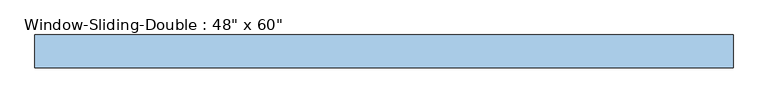
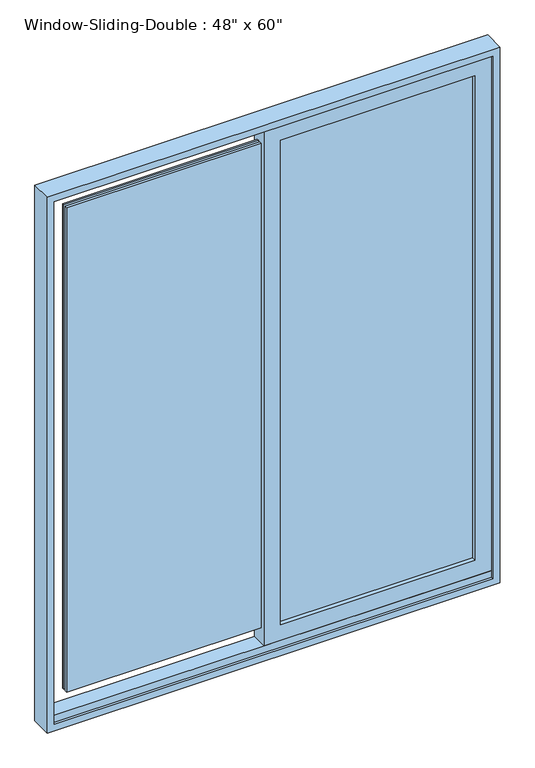
"""IFC4 building model written with IfcOpenShell, lengths in millimetres: window geometry."""

import ifcopenshell
import ifcopenshell.guid

model = None  # the IFC model being written
_history = None  # IfcOwnerHistory: only IFC2X3 demands one
_inside = {}  # id of a spatial element -> (the spatial element, [elements in it])
_under = {}  # id of a project, library or spatial element -> (it, [spatial elements below it])
_declared = {}  # id of a project -> (the project, [libraries it declares])
_typed = {}  # id of a type object -> (the type object, [elements of that type])
_made_of = {}  # id of a material, layer set ... -> (it, [elements and type objects made of it])


def new_model(schema):
    """Start an empty IFC model of exactly this schema.

    Asked for "IFC4X3", IfcOpenShell would pick the latest addendum, in which some entities
    have other attributes; the version numbers below select the first issue.
    IFC2X3 requires an IfcOwnerHistory on every rooted entity: one is made here for all.
    """
    global model, _history
    if schema == "IFC4X3":
        model = ifcopenshell.file(schema_version=(4, 3, 0, 0))
    else:
        model = ifcopenshell.file(schema=schema)
    _inside.clear()
    _under.clear()
    _declared.clear()
    _typed.clear()
    _made_of.clear()
    _history = None
    if model.schema == "IFC2X3":
        org = make("IfcOrganization", Name="unknown")
        user = make(
            "IfcPersonAndOrganization",
            ThePerson=make("IfcPerson", FamilyName="unknown"),
            TheOrganization=org,
        )
        app = make(
            "IfcApplication",
            ApplicationDeveloper=org,
            Version="unknown",
            ApplicationFullName="unknown",
            ApplicationIdentifier="unknown",
        )
        _history = make(
            "IfcOwnerHistory",
            OwningUser=user,
            OwningApplication=app,
            ChangeAction="ADDED",
            CreationDate=0,
        )
    return model


def make(cls, **values):
    """One entity of the class cls with the attributes given. An attribute that is None is left unset."""
    return model.create_entity(
        cls, **{name: value for name, value in values.items() if value is not None}
    )


def rooted(cls, **values):
    """An entity with a GlobalId (a new one), such as an element, a storey or a relation."""
    return make(cls, GlobalId=ifcopenshell.guid.new(), OwnerHistory=_history, **values)


def si_unit(unit_type, name, prefix=None):
    """IfcSIUnit, for example si_unit("LENGTHUNIT", "METRE", prefix="MILLI")."""
    return make("IfcSIUnit", UnitType=unit_type, Prefix=prefix, Name=name)


def assignment(units):
    """IfcUnitAssignment: the units of a project."""
    return None if units is None else make("IfcUnitAssignment", Units=units)


def point(xyz):
    """IfcCartesianPoint."""
    return None if xyz is None else make("IfcCartesianPoint", Coordinates=xyz)


def direction(xyz):
    """IfcDirection."""
    return None if xyz is None else make("IfcDirection", DirectionRatios=xyz)


def frame(location, z_axis=None, x_axis=None):
    """IfcAxis2Placement3D, a coordinate frame: its origin and axes. An axis left out is left unset."""
    return make(
        "IfcAxis2Placement3D",
        Location=point(location),
        Axis=direction(z_axis),
        RefDirection=direction(x_axis),
    )


def origin():
    """The frame at (0, 0, 0) with its axes left unset."""
    return frame((0.0, 0.0, 0.0))


def place(relative_to, where):
    """IfcLocalPlacement: puts the frame where relative to a parent placement (None: the world)."""
    return make(
        "IfcLocalPlacement", PlacementRelTo=relative_to, RelativePlacement=where
    )


def context(
    kind, dimensions, precision=None, world=None, true_north=None, identifier=None
):
    """IfcGeometricRepresentationContext, for example the 3D "Model" context."""
    return make(
        "IfcGeometricRepresentationContext",
        ContextIdentifier=identifier,
        ContextType=kind,
        CoordinateSpaceDimension=dimensions,
        Precision=precision,
        WorldCoordinateSystem=world,
        TrueNorth=true_north,
    )


def project(units=None, contexts=None):
    """IfcProject with its units and contexts."""
    return rooted(
        "IfcProject",
        Name="project",
        RepresentationContexts=contexts,
        UnitsInContext=assignment(units),
    )


def spatial(cls, under=None, at=None, **own):
    """A site, building, storey or space (cls), placed at a placement, below another one or the project."""
    s = rooted(cls, ObjectPlacement=at, **own)
    if under is not None:
        _under.setdefault(under.id(), (under, []))[1].append(s)
    return s


def polyline(points):
    """IfcPolyline through the points."""
    return make("IfcPolyline", Points=[point(p) for p in points])


def outline(outer, holes=None, kind="AREA"):
    """IfcArbitraryClosedProfileDef: a profile drawn as a closed curve; with holes, ...WithVoids."""
    if holes is None:
        return make("IfcArbitraryClosedProfileDef", ProfileType=kind, OuterCurve=outer)
    return make(
        "IfcArbitraryProfileDefWithVoids",
        ProfileType=kind,
        OuterCurve=outer,
        InnerCurves=holes,
    )


def extrude(swept, where, along, depth):
    """IfcExtrudedAreaSolid: the profile swept, set in the frame where, extruded along a direction by depth."""
    return make(
        "IfcExtrudedAreaSolid",
        SweptArea=swept,
        Position=where,
        ExtrudedDirection=direction(along),
        Depth=depth,
    )


def faces_of(points, faces, orient=None, outer=None):
    """IfcFace entities. A face is a list of loops; a loop is a list of indices into points, from 0.

    orient and outer hold one flag for each loop. By default every Orientation is true, the
    first loop of a face is its IfcFaceOuterBound and the others are IfcFaceBound.
    """
    made = []
    for i, loops in enumerate(faces):
        bounds = []
        for j, loop in enumerate(loops):
            is_outer = j == 0 if outer is None else outer[i][j]
            bounds.append(
                make(
                    "IfcFaceOuterBound" if is_outer else "IfcFaceBound",
                    Bound=make("IfcPolyLoop", Polygon=[points[k] for k in loop]),
                    Orientation=True if orient is None else orient[i][j],
                )
            )
        made.append(make("IfcFace", Bounds=bounds))
    return made


def faceted_brep(points, faces, orient=None, outer=None, voids=None):
    """IfcFacetedBrep: a solid bounded by flat faces; with voids (closed shells), ...WithVoids."""
    shared = [point(p) for p in points]
    hull = make("IfcClosedShell", CfsFaces=faces_of(shared, faces, orient, outer))
    if voids is None:
        return make("IfcFacetedBrep", Outer=hull)
    return make(
        "IfcFacetedBrepWithVoids",
        Outer=hull,
        Voids=[
            make(cls, CfsFaces=faces_of(shared, fs, o, b)) for cls, fs, o, b in voids
        ],
    )


def shape(context_of_items, identifier, shape_type, items):
    """IfcShapeRepresentation: the items that make up one representation, for example the "Body"."""
    return make(
        "IfcShapeRepresentation",
        ContextOfItems=context_of_items,
        RepresentationIdentifier=identifier,
        RepresentationType=shape_type,
        Items=items,
    )


def source(mapping_origin, context_of_items, identifier, shape_type, items):
    """IfcRepresentationMap: a shape defined once, which mapped items show again and again."""
    return make(
        "IfcRepresentationMap",
        MappingOrigin=mapping_origin,
        MappedRepresentation=shape(context_of_items, identifier, shape_type, items),
    )


def transform(
    local_origin,
    x_axis=None,
    y_axis=None,
    z_axis=None,
    scale=None,
    scale2=None,
    scale3=None,
    uniform=True,
):
    """IfcCartesianTransformationOperator3D, or its non-uniform kind. x_axis, y_axis, z_axis: its Axis1, 2, 3."""
    if uniform:
        return make(
            "IfcCartesianTransformationOperator3D",
            Axis1=direction(x_axis),
            Axis2=direction(y_axis),
            LocalOrigin=point(local_origin),
            Scale=scale,
            Axis3=direction(z_axis),
        )
    return make(
        "IfcCartesianTransformationOperator3DnonUniform",
        Axis1=direction(x_axis),
        Axis2=direction(y_axis),
        LocalOrigin=point(local_origin),
        Scale=scale,
        Axis3=direction(z_axis),
        Scale2=scale2,
        Scale3=scale3,
    )


def mapped(mapping_source, mapping_target):
    """IfcMappedItem: shows the shape of a source again, moved by a transform."""
    return make(
        "IfcMappedItem", MappingSource=mapping_source, MappingTarget=mapping_target
    )


def made_of(thing, what):
    """Note that an element or type object is made of a material, layer set ...; save() writes the relation."""
    if what is not None:
        _made_of.setdefault(what.id(), (what, []))[1].append(thing)
    return thing


def element(
    cls,
    number,
    at=None,
    inside=None,
    cuts=None,
    type_object=None,
    material=None,
    context=None,
    identifier="Body",
    shape_type=None,
    held_by="IfcProductDefinitionShape",
    body=None,
    shapes=None,
    **own,
):
    """One element of the class cls, such as IfcWall. Its Tag is "e" and its number.

    at: its placement. inside: the storey or other place that contains it. cuts: it is an
    opening in that element (IfcRelVoidsElement). A single representation is given by context,
    identifier, shape_type and body (its items); several are given by shapes. held_by: the class
    of the entity that holds the representations. save() writes the other relations.
    """
    e = rooted(cls, Tag="e%d" % number, ObjectPlacement=at, **own)
    if body is not None:
        shapes = [shape(context, identifier, shape_type, body)]
    if shapes is not None:
        e.Representation = make(held_by, Representations=shapes)
    if inside is not None:
        _inside.setdefault(inside.id(), (inside, []))[1].append(e)
    if cuts is not None:
        rooted(
            "IfcRelVoidsElement", RelatingBuildingElement=cuts, RelatedOpeningElement=e
        )
    if type_object is not None:
        _typed.setdefault(type_object.id(), (type_object, []))[1].append(e)
    return made_of(e, material)


def aggregate(whole, parts):
    """IfcRelAggregates: a whole, such as a stair, and the parts it consists of."""
    return rooted("IfcRelAggregates", RelatingObject=whole, RelatedObjects=parts)


def save(model, path):
    """Write the relations noted so far, then the file.

    IfcRelAggregates (storeys below a building ...), IfcRelContainedInSpatialStructure (elements
    in a storey), IfcRelDefinesByType, IfcRelAssociatesMaterial and IfcRelDeclares: one each for
    every whole, place, type object, material and project.
    """
    for whole, parts in _under.values():
        aggregate(whole, parts)
    for where, things in _inside.values():
        rooted(
            "IfcRelContainedInSpatialStructure",
            RelatedElements=things,
            RelatingStructure=where,
        )
    for kind, things in _typed.values():
        rooted("IfcRelDefinesByType", RelatedObjects=things, RelatingType=kind)
    for what, things in _made_of.values():
        rooted("IfcRelAssociatesMaterial", RelatedObjects=things, RelatingMaterial=what)
    for by, libraries in _declared.values():
        rooted("IfcRelDeclares", RelatingContext=by, RelatedDefinitions=libraries)
    model.write(path)


def window_57c2f901(model_context):
    return source(origin(), model_context, "Body", "SolidModel", [
        faceted_brep([(-609.6, -10.16, 914.4), (-609.6, 46.99, 914.4), (609.6, 46.99, 914.4), (609.6, -10.16, 914.4), (-568.6778905, 46.99, 2397.4778905), (-568.6778905, 40.64, 2397.4778905), (-568.6778905, 40.64, 952.5), (-568.6778905, 40.64, 933.45), (-568.6778905, 46.99, 933.45), (568.6778905, 40.64, 2397.4778905), (568.6778905, 40.64, 952.5), (590.55, 40.64, 952.5), (590.55, 40.64, 2419.35), (-590.55, 40.64, 2419.35), (-590.55, 40.64, 952.5), (-590.55, -10.16, 2419.35), (-590.55, -10.16, 933.45), (-590.55, -3.81, 933.45), (-590.55, -3.81, 952.5), (609.6, -10.16, 2438.4), (-609.6, -10.16, 2438.4), (590.55, -10.16, 2419.35), (590.55, -10.16, 933.45), (-609.6, 46.99, 2438.4), (609.6, 46.99, 2438.4), (568.6778905, 46.99, 933.45), (568.6778905, 46.99, 2397.4778905), (568.6778905, 40.64, 933.45), (590.55, -3.81, 952.5), (590.55, -3.81, 933.45)], [[[0, 1, 2, 3]], [[4, 5, 6, 7, 8]], [[5, 9, 10, 11, 12, 13, 14, 6]], [[13, 15, 16, 17, 18, 14]], [[0, 3, 19, 20], [21, 22, 16, 15]], [[23, 1, 0, 20]], [[2, 1, 23, 24], [4, 8, 25, 26]], [[5, 4, 26, 9]], [[13, 12, 21, 15]], [[20, 19, 24, 23]], [[9, 26, 25, 27, 10]], [[21, 12, 11, 28, 29, 22]], [[19, 3, 2, 24]], [[7, 27, 25, 8]], [[27, 7, 6, 10]], [[10, 6, 14, 18, 28, 11]], [[28, 18, 17, 29]], [[16, 22, 29, 17]]]),
        extrude(outline(polyline([(546.1, 27.94), (546.1, 21.59), (22.225, 21.59), (22.225, 27.94), (546.1, 27.94)])), frame((0.0, 0.0, 996.95), z_axis=(0.0, 0.0, 1.0), x_axis=(1.0, 0.0, 0.0)), (0.0, 0.0, 1.0), 1377.95),
        extrude(outline(polyline([(546.1, 15.24), (546.1, 8.89), (22.225, 8.89), (22.225, 15.24), (546.1, 15.24)])), frame((0.0, 0.0, 996.95), z_axis=(0.0, 0.0, 1.0), x_axis=(1.0, 0.0, 0.0)), (0.0, 0.0, 1.0), 1377.95),
        extrude(outline(polyline([(-22.225, 27.94), (-22.225, 21.59), (-546.1, 21.59), (-546.1, 27.94), (-22.225, 27.94)])), frame((0.0, 0.0, 996.95), z_axis=(0.0, 0.0, 1.0), x_axis=(1.0, 0.0, 0.0)), (0.0, 0.0, 1.0), 1377.95),
        extrude(outline(polyline([(-22.225, 15.24), (-22.225, 8.89), (-546.1, 8.89), (-546.1, 15.24), (-22.225, 15.24)])), frame((0.0, 0.0, 996.95), z_axis=(0.0, 0.0, 1.0), x_axis=(1.0, 0.0, 0.0)), (0.0, 0.0, 1.0), 1377.95),
        extrude(outline(polyline([(952.5, 590.55), (2419.35, 590.55), (2419.35, -22.225), (952.5, -22.225), (952.5, 590.55)]), holes=[polyline([(996.95, 22.225), (2374.9, 22.225), (2374.9, 546.1), (996.95, 546.1), (996.95, 22.225)])]), frame((0.0, -3.81, 0.0), z_axis=(0.0, 1.0, 0.0), x_axis=(0.0, 0.0, 1.0)), (0.0, 0.0, 1.0), 44.45),
    ])


if __name__ == "__main__":
    model = new_model("IFC4")
    model_context = context("Model", 3, world=origin())
    ifc_project = project(units=[si_unit("LENGTHUNIT", "METRE", prefix="MILLI")], contexts=[model_context])
    site = spatial("IfcSite", under=ifc_project)
    building = spatial("IfcBuilding", under=site)
    placement = place(None, origin())
    window_shape = window_57c2f901(model_context)
    element("IfcWindow", 1, ObjectType="Window-Sliding-Double : 48\" x 60\"", at=placement, inside=building, context=model_context, shape_type="MappedRepresentation", body=[
        mapped(window_shape, transform((0.0, 0.0, 0.0), x_axis=(1.0, 0.0, 0.0), y_axis=(0.0, 1.0, 0.0), z_axis=(0.0, 0.0, 1.0))),
    ])
    save(model, "model.ifc")

# Revit data of these elements
# Type "Window-Sliding-Double : 48\" x 60\""
#   Type Mark = "19"
#   Fire Rating = "0.5h"
#   Assembly Code = "B2020100"
#   Analytic Construction = "Double glazing - domestic"
#   Window Inset [instance default] = 0' - 0"
#   Wall Thickness [instance default] = 0' - 6"
#   Visual Light Transmittance = 0.81
#   Thermal Resistance (R) = 1.8146 (h·ft²·°F)/BTU
#   Solar Heat Gain Coefficient = 0.76
#   Muntin Width = 1' - 8 5/8"
#   Muntin Height = 4' - 6 1/4"
#   Interior Wall Closure [instance default] = 0' - 2 3/4"
#   Heat Transfer Coefficient (U) = 0.5511 BTU/(h·ft²·°F)
#   Frame Extension [instance default] = 0' - 0 1/4"
#   Exterior Wall Closure [instance default] = 0' - 1 1/4"
#   Rough Width = 4' - 0 1/2"
#   Rough Height = 5' - 0 1/2"
#   Height = 5' - 0"
#   Extension Jamb [instance default] = 0' - 2 3/4"
#   Default Sill Height = 3' - 0"
#   Width = 4' - 0"
#   Interior Trim Visibility [instance default] = yes
#   Indicator Visibility [instance default] = yes
#   Exterior Trim Visibility [instance default] = yes
#   Muntin Visibility = yes
#   Extension Jamb Visibility [instance default] = yes
#   Muntin Pattern = Muntin Pattern_2x2 : Muntin Pattern_2x2
#   Interior Trim Material = Wood - Stained
#   Interior Trim = Trim-Window-Interior-Flat : Picture Frame
#   Interior Frame Material = Wood - Stained
#   Glass Panel Material = Glass
#   Exterior Trim Material = Clad - White
#   Exterior Trim = Trim-Window-Exterior-Flat : with Sill
#   Exterior Frame Material = Clad - White
#   Wall Closure = (empty or 0)
# Element 1 (IfcWindow, "Window-Sliding-Double : 48\" x 60\"")
#   Wall Thickness = 0' - 2 1/2"
#   Extension Jamb = 0' - 1"
#   Extension Jamb Visibility = no
#   Materials on its faces: "Glass", "Wood - Stained", "Clad - White"
# Materials
#   "Wood - Stained": class "Wood", colour RGB 224 178 126, transparency 0, Cost = 0
#   "Glass": class "Glass", colour RGB 0 128 192, transparency 0.75, Description = "Soda Lime Glass", Cost = 0
#   "Clad - White": class "Wood", colour RGB 242 242 238, transparency 0, Cost = 0
